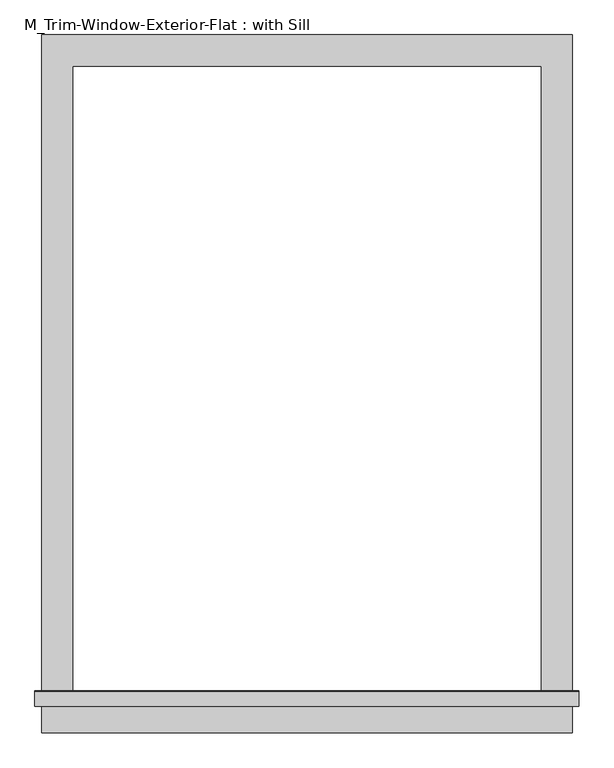
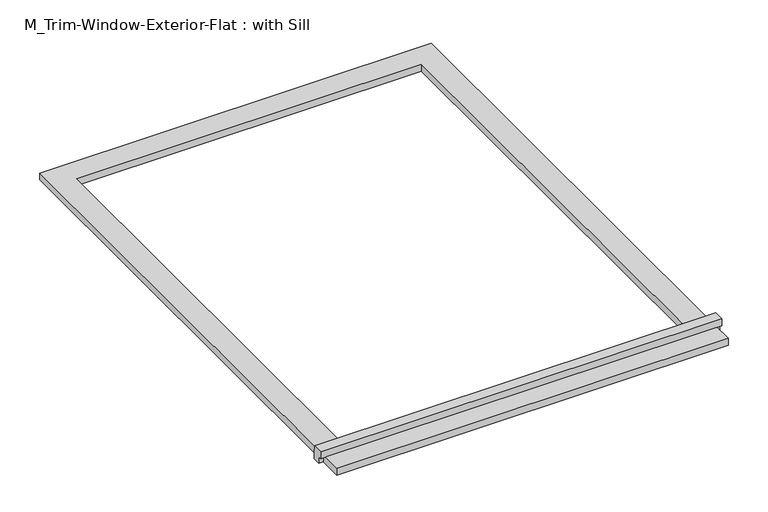
"""IFC4 building model written with IfcOpenShell, lengths in millimetres: proxy geometry, M_Trim-Window-Exterior-Flat : with Sill."""

from ifc_helpers import new_model, si_unit, frame, origin, origin_with_axes, place, context, project, spatial, polyline, outline, extrude, source, transform, mapped, element, save


def m_trim_window_exterior_flat_with_sill_71544b40(model_context):
    return source(origin(), model_context, "Body", "SweptSolid", [
        extrude(outline(polyline([(510.0, -1220.4323709), (510.0, -1280.4323709), (-510.0, -1280.4323709), (-510.0, -1220.4323709), (510.0, -1220.4323709)])), origin_with_axes(), (0.0, 0.0, 1.0), 19.05),
        extrude(outline(polyline([(-1230.0, 38.1), (-1202.4580645, 38.1), (-1200.0, 19.05), (-1200.0, 0.0), (-1220.4323709, 0.0), (-1220.4323709, 19.05), (-1230.0, 19.05), (-1230.0, 38.1)])), frame((-522.7, 0.0, 0.0), z_axis=(1.0, 0.0, 0.0), x_axis=(0.0, 1.0, 0.0)), (0.0, 0.0, 1.0), 1045.4),
        extrude(outline(polyline([(-510.0, 60.0), (510.0, 60.0), (510.0, -1200.0), (450.0, -1200.0), (450.0, 0.0), (-450.0, 0.0), (-450.0, -1200.0), (-510.0, -1200.0), (-510.0, 60.0)])), origin_with_axes(), (0.0, 0.0, 1.0), 19.05),
    ])


if __name__ == "__main__":
    model = new_model("IFC4")
    model_context = context("Model", 3, world=origin())
    ifc_project = project(units=[si_unit("LENGTHUNIT", "METRE", prefix="MILLI")], contexts=[model_context])
    site = spatial("IfcSite", under=ifc_project)
    building = spatial("IfcBuilding", under=site)
    placement = place(None, origin())
    m_trim_window_exterior_flat_with_sill_shape = m_trim_window_exterior_flat_with_sill_71544b40(model_context)
    element("IfcBuildingElementProxy", 1, Name="M_Trim-Window-Exterior-Flat : with Sill", ObjectType="M_Trim-Window-Exterior-Flat : with Sill", at=placement, inside=building, context=model_context, shape_type="MappedRepresentation", body=[
        mapped(m_trim_window_exterior_flat_with_sill_shape, transform((0.0, 0.0, 0.0), x_axis=(1.0, 0.0, 0.0), y_axis=(0.0, 1.0, 0.0), z_axis=(0.0, 0.0, 1.0))),
    ])
    save(model, "model.ifc")

# Revit data of these elements
# Type "M_Trim-Window-Exterior-Flat : with Sill"
#   Trim Width = 60 mm
#   Trim Thickness_Picture Frame = 30 mm
#   Trim Thickness_with Sill = 19.05 mm
#   Sill Thickness = 30 mm
#   Opening Width [instance default] = 600 mm
#   Opening Height [instance default] = 900 mm
#   Default Elevation = 1200 mm
#   Sill = yes
#   Picture Frame = no
#   Trim Material [instance default] = none
# Element 1 (IfcBuildingElementProxy, "M_Trim-Window-Exterior-Flat : with Sill")
#   Opening Width = 900 mm
#   Opening Height = 1200 mm
#   Trim Material = Clad - White
#   Materials on its faces: "Clad - White"
# Materials
#   "Clad - White": class "Wood", colour RGB 245 245 243, transparency 0, Cost = 0
